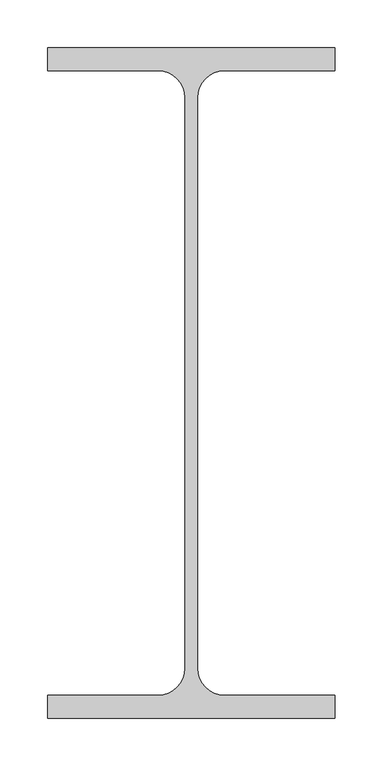
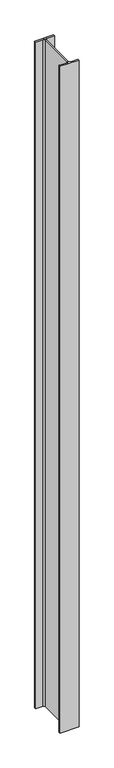
"""IFC4 building model written with IfcOpenShell, lengths in millimetres: column geometry, 0912_Steel Column_H_KSD3502 : H_SC_ASC_H-700x300x13x24."""

from ifc_helpers import new_model, si_unit, point, frame_2d, origin, origin_with_axes, place, context, project, spatial, polyline, circle_curve, trimmed, segment, composite_curve, outline, extrude, source, transform, mapped, element, save


def column_ca8bed04(model_context):
    return source(origin(), model_context, "Body", "SweptSolid", [
        extrude(outline(composite_curve([segment(polyline([(150.0, 350.0), (150.0, 326.0), (34.5, 326.0)]), True, "CONTINUOUS"), segment(trimmed(circle_curve(frame_2d((34.5, 298.0)), 28.0), [point((34.5, 326.0))], [point((6.5, 298.0))], True, "CARTESIAN"), True, "CONTINUOUS"), segment(polyline([(6.5, 298.0), (6.5, -298.0)]), True, "CONTINUOUS"), segment(trimmed(circle_curve(frame_2d((34.5, -298.0)), 28.0), [point((6.5, -298.0))], [point((34.5, -326.0))], True, "CARTESIAN"), True, "CONTINUOUS"), segment(polyline([(34.5, -326.0), (150.0, -326.0), (150.0, -350.0), (-150.0, -350.0), (-150.0, -326.0), (-34.5, -326.0)]), True, "CONTINUOUS"), segment(trimmed(circle_curve(frame_2d((-34.5, -298.0)), 28.0), [point((-34.5, -326.0))], [point((-6.5, -298.0))], True, "CARTESIAN"), True, "CONTINUOUS"), segment(polyline([(-6.5, -298.0), (-6.5, 298.0)]), True, "CONTINUOUS"), segment(trimmed(circle_curve(frame_2d((-34.5, 298.0)), 28.0), [point((-6.5, 298.0))], [point((-34.5, 326.0))], True, "CARTESIAN"), True, "CONTINUOUS"), segment(polyline([(-34.5, 326.0), (-150.0, 326.0), (-150.0, 350.0), (150.0, 350.0)]), True, "CONTINUOUS")], self_intersect=False)), origin_with_axes(), (0.0, 0.0, 1.0), 11224.0),
    ])


if __name__ == "__main__":
    model = new_model("IFC4")
    model_context = context("Model", 3, world=origin())
    ifc_project = project(units=[si_unit("LENGTHUNIT", "METRE", prefix="MILLI")], contexts=[model_context])
    site = spatial("IfcSite", under=ifc_project)
    building = spatial("IfcBuilding", under=site)
    placement = place(None, origin())
    column_shape = column_ca8bed04(model_context)
    element("IfcColumn", 1, ObjectType="0912_Steel Column_H_KSD3502 : H_SC_ASC_H-700x300x13x24", at=placement, inside=building, context=model_context, shape_type="MappedRepresentation", body=[
        mapped(column_shape, transform((0.0, 0.0, 0.0), x_axis=(1.0, 0.0, 0.0), y_axis=(0.0, 1.0, 0.0), z_axis=(0.0, 0.0, 1.0))),
    ])
    save(model, "model.ifc")

# Revit data of these elements
# Type "0912_Steel Column_H_KSD3502 : H_SC_ASC_H-700x300x13x24"
#   H_WM Code_1 = "S01AA002-00001 | Main Steel Structure Fabrication Work | Shelter/Building | Medium Steel - Standard (90KG/M>Weight≥30KG/M) | Material: (   )"
#   H_WM Code_2 = "S03AA028-00001 | Main Steel Structure Erection Work | Shelter/Building | Medium Steel (90KG/M>Weight≥30KG/M) | Material: (   )"
#   H_WM Code_3 = "S01AA010-00001 | Main Steel Structure Fabrication Work | Shelter/Building | Steel Painting/Coating | for Non-Fireproofed Steel Surface, Surface Preparation, Primer, Second & Final Coat | Material: (   )"
#   H_Q'ty Cal Type Tag = "SC-Q2"
#   Width = 30.0 cm
#   Web Thickness = 1.3 cm
#   Web Fillet = 2.8 cm
#   Warping Constant = 12338400.0 cm⁶
#   Torsional Moment of Inertia = 325.986 cm⁴
#   Section Area = 235.5 cm²
#   Plastic Modulus weak axis = 1120.0 cm³
#   Plastic Modulus strong axis = 6460.0 cm³
#   Perimeter = 2.53 m²/m
#   Nominal Weight = 185.00 kgf/m
#   Moment of Inertia weak axis = 10800.00 cm⁴
#   Moment of Inertia strong axis = 201000.00 cm⁴
#   Height = 70.0 cm
#   Flange Thickness = 2.4 cm
#   Elastic Modulus weak axis = 722.0 cm³
#   Elastic Modulus strong axis = 5760.0 cm³
#   Centroid Vertical = 35.0 cm
#   Centroid Horizontal = 15.0 cm
#   Structural Material [instance default] = Steel, 45-345
#   Section Name Key = ""
#   Bolt Spacing = 0
#   Assembly Code = ""
# Element 1 (IfcColumn, "0912_Steel Column_H_KSD3502 : H_SC_ASC_H-700x300x13x24")
#   Structural Material = A03AD029-00008_Anchor Bolt (Installation only)_M36
#   Materials on its faces: "A03AD029-00008_Anchor Bolt (Installation only)_M36"
# Materials
#   "Steel, 45-345": class "Metal", colour RGB 189 187 185, transparency 0, Description = "Steel 345 MPa", Cost = 0
#   "A03AD029-00008_Anchor Bolt (Installation only)_M36": class "Unassigned", colour RGB 84 83 81, transparency 0, Cost = 0
